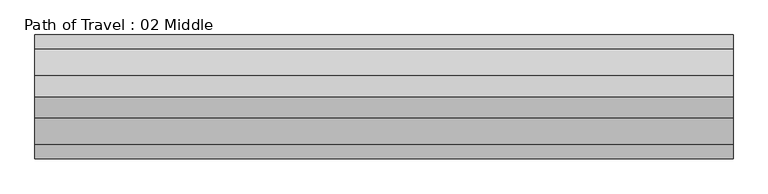
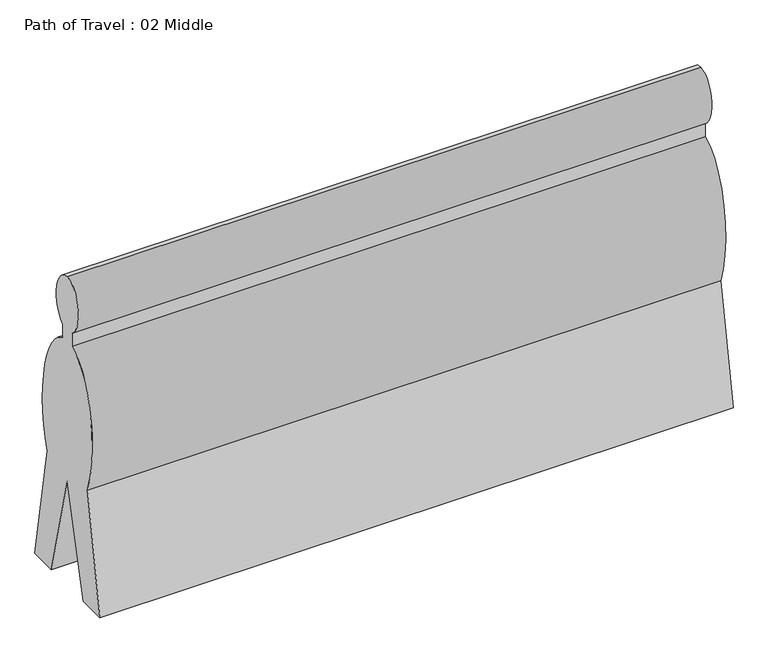
"""IFC4 building model written with IfcOpenShell, lengths in millimetres: proxy geometry, Path of Travel : 02 Middle."""

import ifcopenshell
import ifcopenshell.guid

model = None  # the IFC model being written
_history = None  # IfcOwnerHistory: only IFC2X3 demands one
_inside = {}  # id of a spatial element -> (the spatial element, [elements in it])
_under = {}  # id of a project, library or spatial element -> (it, [spatial elements below it])
_declared = {}  # id of a project -> (the project, [libraries it declares])
_typed = {}  # id of a type object -> (the type object, [elements of that type])
_made_of = {}  # id of a material, layer set ... -> (it, [elements and type objects made of it])


def new_model(schema):
    """Start an empty IFC model of exactly this schema.

    Asked for "IFC4X3", IfcOpenShell would pick the latest addendum, in which some entities
    have other attributes; the version numbers below select the first issue.
    IFC2X3 requires an IfcOwnerHistory on every rooted entity: one is made here for all.
    """
    global model, _history
    if schema == "IFC4X3":
        model = ifcopenshell.file(schema_version=(4, 3, 0, 0))
    else:
        model = ifcopenshell.file(schema=schema)
    _inside.clear()
    _under.clear()
    _declared.clear()
    _typed.clear()
    _made_of.clear()
    _history = None
    if model.schema == "IFC2X3":
        org = make("IfcOrganization", Name="unknown")
        user = make(
            "IfcPersonAndOrganization",
            ThePerson=make("IfcPerson", FamilyName="unknown"),
            TheOrganization=org,
        )
        app = make(
            "IfcApplication",
            ApplicationDeveloper=org,
            Version="unknown",
            ApplicationFullName="unknown",
            ApplicationIdentifier="unknown",
        )
        _history = make(
            "IfcOwnerHistory",
            OwningUser=user,
            OwningApplication=app,
            ChangeAction="ADDED",
            CreationDate=0,
        )
    return model


def make(cls, **values):
    """One entity of the class cls with the attributes given. An attribute that is None is left unset."""
    return model.create_entity(
        cls, **{name: value for name, value in values.items() if value is not None}
    )


def rooted(cls, **values):
    """An entity with a GlobalId (a new one), such as an element, a storey or a relation."""
    return make(cls, GlobalId=ifcopenshell.guid.new(), OwnerHistory=_history, **values)


def si_unit(unit_type, name, prefix=None):
    """IfcSIUnit, for example si_unit("LENGTHUNIT", "METRE", prefix="MILLI")."""
    return make("IfcSIUnit", UnitType=unit_type, Prefix=prefix, Name=name)


def assignment(units):
    """IfcUnitAssignment: the units of a project."""
    return None if units is None else make("IfcUnitAssignment", Units=units)


def point(xyz):
    """IfcCartesianPoint."""
    return None if xyz is None else make("IfcCartesianPoint", Coordinates=xyz)


def direction(xyz):
    """IfcDirection."""
    return None if xyz is None else make("IfcDirection", DirectionRatios=xyz)


def frame(location, z_axis=None, x_axis=None):
    """IfcAxis2Placement3D, a coordinate frame: its origin and axes. An axis left out is left unset."""
    return make(
        "IfcAxis2Placement3D",
        Location=point(location),
        Axis=direction(z_axis),
        RefDirection=direction(x_axis),
    )


def origin():
    """The frame at (0, 0, 0) with its axes left unset."""
    return frame((0.0, 0.0, 0.0))


def place(relative_to, where):
    """IfcLocalPlacement: puts the frame where relative to a parent placement (None: the world)."""
    return make(
        "IfcLocalPlacement", PlacementRelTo=relative_to, RelativePlacement=where
    )


def context(
    kind, dimensions, precision=None, world=None, true_north=None, identifier=None
):
    """IfcGeometricRepresentationContext, for example the 3D "Model" context."""
    return make(
        "IfcGeometricRepresentationContext",
        ContextIdentifier=identifier,
        ContextType=kind,
        CoordinateSpaceDimension=dimensions,
        Precision=precision,
        WorldCoordinateSystem=world,
        TrueNorth=true_north,
    )


def project(units=None, contexts=None):
    """IfcProject with its units and contexts."""
    return rooted(
        "IfcProject",
        Name="project",
        RepresentationContexts=contexts,
        UnitsInContext=assignment(units),
    )


def spatial(cls, under=None, at=None, **own):
    """A site, building, storey or space (cls), placed at a placement, below another one or the project."""
    s = rooted(cls, ObjectPlacement=at, **own)
    if under is not None:
        _under.setdefault(under.id(), (under, []))[1].append(s)
    return s


def ellipse_curve(where, semi_axis1, semi_axis2):
    """IfcEllipse in the frame where."""
    return make(
        "IfcEllipse", Position=where, SemiAxis1=semi_axis1, SemiAxis2=semi_axis2
    )


def trimmed(basis, trim1, trim2, sense, master):
    """IfcTrimmedCurve: the piece of a basis curve between two trims."""
    return make(
        "IfcTrimmedCurve",
        BasisCurve=basis,
        Trim1=trim1,
        Trim2=trim2,
        SenseAgreement=sense,
        MasterRepresentation=master,
    )


def shape(context_of_items, identifier, shape_type, items):
    """IfcShapeRepresentation: the items that make up one representation, for example the "Body"."""
    return make(
        "IfcShapeRepresentation",
        ContextOfItems=context_of_items,
        RepresentationIdentifier=identifier,
        RepresentationType=shape_type,
        Items=items,
    )


def source(mapping_origin, context_of_items, identifier, shape_type, items):
    """IfcRepresentationMap: a shape defined once, which mapped items show again and again."""
    return make(
        "IfcRepresentationMap",
        MappingOrigin=mapping_origin,
        MappedRepresentation=shape(context_of_items, identifier, shape_type, items),
    )


def transform(
    local_origin,
    x_axis=None,
    y_axis=None,
    z_axis=None,
    scale=None,
    scale2=None,
    scale3=None,
    uniform=True,
):
    """IfcCartesianTransformationOperator3D, or its non-uniform kind. x_axis, y_axis, z_axis: its Axis1, 2, 3."""
    if uniform:
        return make(
            "IfcCartesianTransformationOperator3D",
            Axis1=direction(x_axis),
            Axis2=direction(y_axis),
            LocalOrigin=point(local_origin),
            Scale=scale,
            Axis3=direction(z_axis),
        )
    return make(
        "IfcCartesianTransformationOperator3DnonUniform",
        Axis1=direction(x_axis),
        Axis2=direction(y_axis),
        LocalOrigin=point(local_origin),
        Scale=scale,
        Axis3=direction(z_axis),
        Scale2=scale2,
        Scale3=scale3,
    )


def mapped(mapping_source, mapping_target):
    """IfcMappedItem: shows the shape of a source again, moved by a transform."""
    return make(
        "IfcMappedItem", MappingSource=mapping_source, MappingTarget=mapping_target
    )


def made_of(thing, what):
    """Note that an element or type object is made of a material, layer set ...; save() writes the relation."""
    if what is not None:
        _made_of.setdefault(what.id(), (what, []))[1].append(thing)
    return thing


def element(
    cls,
    number,
    at=None,
    inside=None,
    cuts=None,
    type_object=None,
    material=None,
    context=None,
    identifier="Body",
    shape_type=None,
    held_by="IfcProductDefinitionShape",
    body=None,
    shapes=None,
    **own,
):
    """One element of the class cls, such as IfcWall. Its Tag is "e" and its number.

    at: its placement. inside: the storey or other place that contains it. cuts: it is an
    opening in that element (IfcRelVoidsElement). A single representation is given by context,
    identifier, shape_type and body (its items); several are given by shapes. held_by: the class
    of the entity that holds the representations. save() writes the other relations.
    """
    e = rooted(cls, Tag="e%d" % number, ObjectPlacement=at, **own)
    if body is not None:
        shapes = [shape(context, identifier, shape_type, body)]
    if shapes is not None:
        e.Representation = make(held_by, Representations=shapes)
    if inside is not None:
        _inside.setdefault(inside.id(), (inside, []))[1].append(e)
    if cuts is not None:
        rooted(
            "IfcRelVoidsElement", RelatingBuildingElement=cuts, RelatedOpeningElement=e
        )
    if type_object is not None:
        _typed.setdefault(type_object.id(), (type_object, []))[1].append(e)
    return made_of(e, material)


def aggregate(whole, parts):
    """IfcRelAggregates: a whole, such as a stair, and the parts it consists of."""
    return rooted("IfcRelAggregates", RelatingObject=whole, RelatedObjects=parts)


def save(model, path):
    """Write the relations noted so far, then the file.

    IfcRelAggregates (storeys below a building ...), IfcRelContainedInSpatialStructure (elements
    in a storey), IfcRelDefinesByType, IfcRelAssociatesMaterial and IfcRelDeclares: one each for
    every whole, place, type object, material and project.
    """
    for whole, parts in _under.values():
        aggregate(whole, parts)
    for where, things in _inside.values():
        rooted(
            "IfcRelContainedInSpatialStructure",
            RelatedElements=things,
            RelatingStructure=where,
        )
    for kind, things in _typed.values():
        rooted("IfcRelDefinesByType", RelatedObjects=things, RelatingType=kind)
    for what, things in _made_of.values():
        rooted("IfcRelAssociatesMaterial", RelatedObjects=things, RelatingMaterial=what)
    for by, libraries in _declared.values():
        rooted("IfcRelDeclares", RelatingContext=by, RelatedDefinitions=libraries)
    model.write(path)


def plane_surface(at):
    """IfcPlane: the flat surface through the origin of the frame at, square to its z axis."""
    return make("IfcPlane", Position=at)


def extruded_surface(curve, direction_of_extrusion, depth):
    """IfcSurfaceOfLinearExtrusion: the curve pushed along a direction by depth."""
    return make(
        "IfcSurfaceOfLinearExtrusion",
        SweptCurve=make("IfcArbitraryOpenProfileDef", ProfileType="CURVE", Curve=curve),
        ExtrudedDirection=direction(direction_of_extrusion),
        Depth=depth,
    )


def advanced_brep(points, edges, surfaces, faces):
    """IfcAdvancedBrep: a solid bounded by faces that lie on surfaces and meet in shared edges.

    An edge is (start, end): straight between two places in points (the first is 0);
    or (start, end, curve); or (start, end, curve, False) where it runs against its curve.
    A face is (place in surfaces, loops), or (place, loops, False) where it looks against
    its surface's normal. A loop lists edges by number (the first is 1), with a minus sign
    where the edge is run from its end to its start. The first loop is the outer one.
    """
    corners = [point(p) for p in points]
    vertices = [make("IfcVertexPoint", VertexGeometry=c) for c in corners]
    made = []
    for start, end, *more in edges:
        made.append(
            make(
                "IfcEdgeCurve",
                EdgeStart=vertices[start],
                EdgeEnd=vertices[end],
                EdgeGeometry=more[0] if more else make("IfcPolyline", Points=[corners[start], corners[end]]),
                SameSense=more[1] if len(more) > 1 else True,
            )
        )
    hull = []
    for where, loops, *sense in faces:
        bounds = []
        for j, loop in enumerate(loops):
            ring = [make("IfcOrientedEdge", EdgeElement=made[abs(k) - 1], Orientation=k > 0) for k in loop]
            bounds.append(
                make(
                    "IfcFaceOuterBound" if j == 0 else "IfcFaceBound",
                    Bound=make("IfcEdgeLoop", EdgeList=ring),
                    Orientation=True,
                )
            )
        hull.append(make("IfcAdvancedFace", Bounds=bounds, FaceSurface=surfaces[where], SameSense=sense[0] if sense else True))
    return make("IfcAdvancedBrep", Outer=make("IfcClosedShell", CfsFaces=hull))


def path_of_travel_02_middle_3bd4d48d(model_context):
    return source(origin(), model_context, "Body", "AdvancedBrep", [
        advanced_brep(
        [(227.5554837, 0.0, 1727.2), (227.5554837, 42.9018657, 1436.6534209), (227.5554837, 42.9018657, 1363.4763406), (227.5554837, 184.1186263, 643.4144547), (227.5554837, 297.5699544, 0.0), (227.5554837, 145.6574193, 0.0), (227.5554837, 0.0, 584.2), (227.5554837, -145.6574193, 0.0), (227.5554837, -297.5699544, 0.0), (227.5554837, -184.1186263, 643.4144547), (227.5554837, -42.9018657, 1363.4763406), (227.5554837, -42.9018657, 1436.6534209), (3580.3554837, 0.0, 1727.2), (3580.3554837, -42.9018657, 1436.6534209), (3580.3554837, -42.9018657, 1363.4763406), (3580.3554837, -184.1186263, 643.4144547), (3580.3554837, -297.5699544, 0.0), (3580.3554837, -145.6574193, 0.0), (3580.3554837, 0.0, 584.2), (3580.3554837, 145.6574193, 0.0), (3580.3554837, 297.5699544, 0.0), (3580.3554837, 184.1186263, 643.4144547), (3580.3554837, 42.9018657, 1363.4763406), (3580.3554837, 42.9018657, 1436.6534209)],
        [
            (0, 1, ellipse_curve(frame((227.5554837, 0.0, 1574.8), z_axis=(-1.0, 0.0, 0.0), x_axis=(0.0, 0.0, 1.0)), 152.4, 101.6)),
            (1, 2),
            (2, 3, ellipse_curve(frame((227.5554837, 0.0, 914.4), z_axis=(-1.0, 0.0, 0.0), x_axis=(0.0, 0.0, -1.0)), 457.2, 228.6)),
            (3, 4),
            (4, 5),
            (5, 6),
            (6, 7),
            (7, 8),
            (8, 9),
            (9, 10, ellipse_curve(frame((227.5554837, 0.0, 914.4), z_axis=(-1.0, 0.0, 0.0), x_axis=(0.0, 0.0, -1.0)), 457.2, 228.6)),
            (10, 11),
            (11, 0, ellipse_curve(frame((227.5554837, 0.0, 1574.8), z_axis=(-1.0, 0.0, 0.0), x_axis=(0.0, 0.0, 1.0)), 152.4, 101.6)),
            (12, 13, ellipse_curve(frame((3580.3554837, 0.0, 1574.8), z_axis=(1.0, 0.0, 0.0), x_axis=(0.0, 0.0, 1.0)), 152.4, 101.6)),
            (13, 14),
            (14, 15, ellipse_curve(frame((3580.3554837, 0.0, 914.4), z_axis=(1.0, 0.0, 0.0), x_axis=(0.0, 0.0, -1.0)), 457.2, 228.6)),
            (15, 16),
            (16, 17),
            (17, 18),
            (18, 19),
            (19, 20),
            (20, 21),
            (21, 22, ellipse_curve(frame((3580.3554837, 0.0, 914.4), z_axis=(1.0, 0.0, 0.0), x_axis=(0.0, 0.0, -1.0)), 457.2, 228.6)),
            (22, 23),
            (23, 12, ellipse_curve(frame((3580.3554837, 0.0, 1574.8), z_axis=(1.0, 0.0, 0.0), x_axis=(0.0, 0.0, 1.0)), 152.4, 101.6)),
            (0, 12),
            (23, 1),
            (22, 2),
            (21, 3),
            (20, 4),
            (19, 5),
            (18, 6),
            (17, 7),
            (16, 8),
            (15, 9),
            (14, 10),
            (13, 11),
        ],
        [
            plane_surface(frame((227.5554837, 0.0, 0.0), z_axis=(-1.0, 0.0, 0.0), x_axis=(0.0, 0.0, 1.0))),
            plane_surface(frame((3580.3554837, 0.0, 0.0), z_axis=(1.0, 0.0, 0.0), x_axis=(0.0, 0.0, 1.0))),
            extruded_surface(trimmed(ellipse_curve(frame((3580.3554837, 0.0, 1574.8), z_axis=(-1.0, 0.0, 0.0), x_axis=(0.0, 0.0, 1.0)), 152.4, 101.6), [point((3580.3554837, 0.0, 1727.2))], [point((3580.3554837, 42.9018657, 1436.6534209))], True, "CARTESIAN"), (-3352.8, 0.0, 0.0), 3352.8),
            plane_surface(frame((227.5554837, 42.9018657, 1436.6534209), z_axis=(0.0, 1.0, 0.0), x_axis=(1.0, 0.0, 0.0))),
            extruded_surface(trimmed(ellipse_curve(frame((3580.3554837, 0.0, 914.4), z_axis=(-1.0, 0.0, 0.0), x_axis=(0.0, 0.0, -1.0)), 457.2, 228.6), [point((3580.3554837, 42.9018657, 1363.4763406))], [point((3580.3554837, 184.1186263, 643.4144547))], True, "CARTESIAN"), (-3352.8, 0.0, 0.0), 3352.8),
            plane_surface(frame((227.5554837, 184.1186263, 643.4144547), z_axis=(0.0, 0.9848077530122078, 0.17364817766693205), x_axis=(1.0, 0.0, 0.0))),
            plane_surface(frame((227.5554837, 297.5699544, 0.0), z_axis=(0.0, 0.0, -1.0), x_axis=(1.0, 0.0, 0.0))),
            plane_surface(frame((227.5554837, 145.6574193, 0.0), z_axis=(0.0, -0.9702957262760199, -0.2419218955995739), x_axis=(1.0, 0.0, 0.0))),
            plane_surface(frame((227.5554837, 0.0, 584.2), z_axis=(0.0, 0.9702957262759961, -0.24192189559966923), x_axis=(1.0, 0.0, 0.0))),
            plane_surface(frame((227.5554837, -145.6574193, 0.0), z_axis=(0.0, 0.0, -1.0), x_axis=(1.0, 0.0, 0.0))),
            plane_surface(frame((227.5554837, -297.5699544, 0.0), z_axis=(0.0, -0.984807753012208, 0.17364817766693066), x_axis=(1.0, 0.0, 0.0))),
            extruded_surface(trimmed(ellipse_curve(frame((3580.3554837, 0.0, 914.4), z_axis=(-1.0, 0.0, 0.0), x_axis=(0.0, 0.0, -1.0)), 457.2, 228.6), [point((3580.3554837, -184.1186263, 643.4144547))], [point((3580.3554837, -42.9018657, 1363.4763406))], True, "CARTESIAN"), (-3352.8, 0.0, 0.0), 3352.8),
            plane_surface(frame((227.5554837, -42.9018657, 1363.4763406), z_axis=(0.0, -1.0, 0.0), x_axis=(1.0, 0.0, 0.0))),
            extruded_surface(trimmed(ellipse_curve(frame((3580.3554837, 0.0, 1574.8), z_axis=(-1.0, 0.0, 0.0), x_axis=(0.0, 0.0, 1.0)), 152.4, 101.6), [point((3580.3554837, -42.9018657, 1436.6534209))], [point((3580.3554837, 0.0, 1727.2))], True, "CARTESIAN"), (-3352.8, 0.0, 0.0), 3352.8),
        ],
        [
            (0, [[1, 2, 3, 4, 5, 6, 7, 8, 9, 10, 11, 12]]),
            (1, [[13, 14, 15, 16, 17, 18, 19, 20, 21, 22, 23, 24]]),
            (2, [[-1, 25, -24, 26]]),
            (3, [[-2, -26, -23, 27]]),
            (4, [[-3, -27, -22, 28]]),
            (5, [[-4, -28, -21, 29]]),
            (6, [[-5, -29, -20, 30]]),
            (7, [[-6, -30, -19, 31]]),
            (8, [[-7, -31, -18, 32]]),
            (9, [[-8, -32, -17, 33]]),
            (10, [[-9, -33, -16, 34]]),
            (11, [[-10, -34, -15, 35]]),
            (12, [[-11, -35, -14, 36]]),
            (13, [[-12, -36, -13, -25]]),
        ],
    ),
    ])


if __name__ == "__main__":
    model = new_model("IFC4")
    model_context = context("Model", 3, world=origin())
    ifc_project = project(units=[si_unit("LENGTHUNIT", "METRE", prefix="MILLI")], contexts=[model_context])
    site = spatial("IfcSite", under=ifc_project)
    building = spatial("IfcBuilding", under=site)
    placement = place(None, origin())
    path_of_travel_02_middle_shape = path_of_travel_02_middle_3bd4d48d(model_context)
    element("IfcBuildingElementProxy", 1, Name="Path of Travel : 02 Middle", ObjectType="Path of Travel : 02 Middle", at=placement, inside=building, context=model_context, shape_type="MappedRepresentation", body=[
        mapped(path_of_travel_02_middle_shape, transform((0.0, 0.0, 0.0), x_axis=(1.0, 0.0, 0.0), y_axis=(0.0, 1.0, 0.0), z_axis=(0.0, 0.0, 1.0))),
    ])
    save(model, "model.ifc")

# Revit data of these elements
# Type "Path of Travel : 02 Middle"
#   Path of Egress [instance default] = 4' - 0"
#   built-in parameter 1001306 [instance default] = 4 (stored number, unit not read)
#   Dot at Start = no
#   Arrow in Middle = yes
#   Arrow at End = no
#   Egress Path = none
# Element 1 (IfcBuildingElementProxy, "Path of Travel : 02 Middle")
#   Path of Egress = 11' - 0"
#   built-in parameter 1001306 = 11 (stored number, unit not read)
#   Materials on its faces: "Egress Path Solid"
# Materials
#   "Egress Path Solid": class "Unassigned", colour RGB 255 128 64, transparency 0.75, Comments = "Rendering appearance not upgraded "
